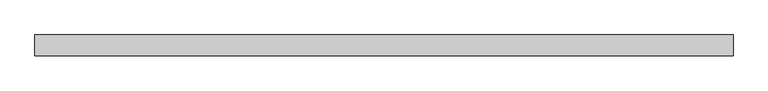
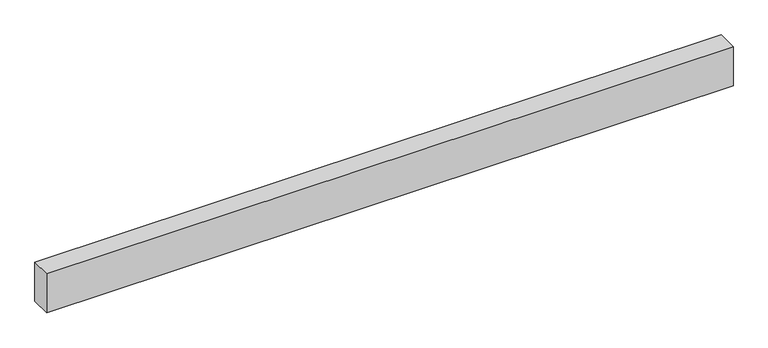
"""IFC4 building model written with IfcOpenShell, lengths in millimetres: beam geometry, Madeira de lei : Berço 6x12cm."""

from ifc_helpers import new_model, si_unit, frame, origin, place, context, project, spatial, polyline, outline, extrude, source, transform, mapped, element, save


def beam_fe4ddbad(model_context):
    return source(origin(), model_context, "Body", "SweptSolid", [
        extrude(outline(polyline([(998.8971968, 30.0), (998.8971968, -30.0), (-998.8971974, -30.0), (-998.8971974, 30.0), (998.8971968, 30.0)])), frame((0.0, 0.0, -60.0), z_axis=(0.0, 0.0, 1.0), x_axis=(1.0, 0.0, 0.0)), (0.0, 0.0, 1.0), 120.0),
    ])


if __name__ == "__main__":
    model = new_model("IFC4")
    model_context = context("Model", 3, world=origin())
    ifc_project = project(units=[si_unit("LENGTHUNIT", "METRE", prefix="MILLI")], contexts=[model_context])
    site = spatial("IfcSite", under=ifc_project)
    building = spatial("IfcBuilding", under=site)
    placement = place(None, origin())
    beam_shape = beam_fe4ddbad(model_context)
    element("IfcBeam", 1, ObjectType="Madeira de lei : Berço 6x12cm", at=placement, inside=building, context=model_context, shape_type="MappedRepresentation", body=[
        mapped(beam_shape, transform((0.0, 0.0, 0.0), x_axis=(1.0, 0.0, 0.0), y_axis=(0.0, 1.0, 0.0), z_axis=(0.0, 0.0, 1.0))),
    ])
    save(model, "model.ifc")

# Revit data of these elements
# Type "Madeira de lei : Berço 6x12cm"
#   A = 0.02 m²
#   Length [instance default] = 1.524 m
#   b = 0.06 m
#   d = 0.12 m
#   Structural Material [instance default] = none
#   Assembly Code = ""
# Element 1 (IfcBeam, "Madeira de lei : Berço 6x12cm")
#   Structural Material = .MADEIRAMENTO
#   Materials on its faces: ".MADEIRAMENTO"
# Materials
#   ".MADEIRAMENTO": class ".CC_MADEIRAS", colour RGB 212 179 113, transparency 0, Cost = 0
